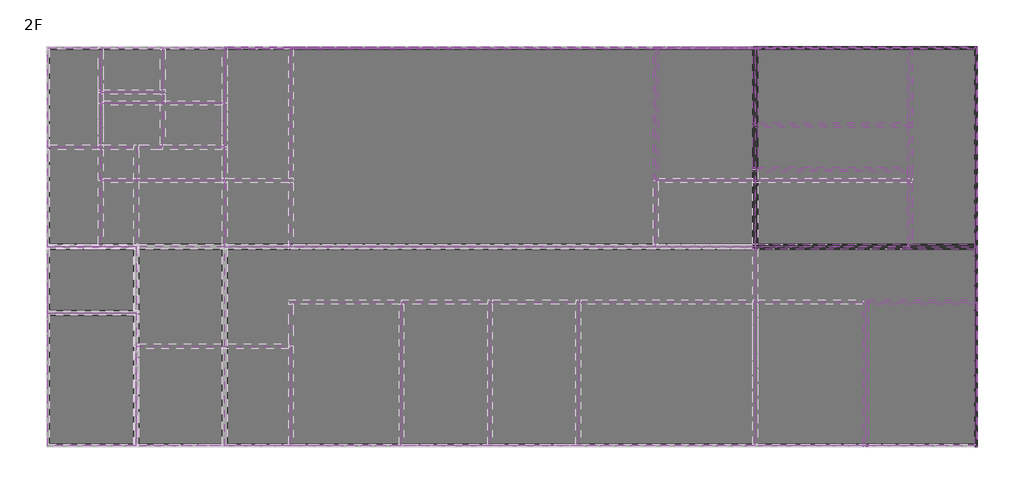
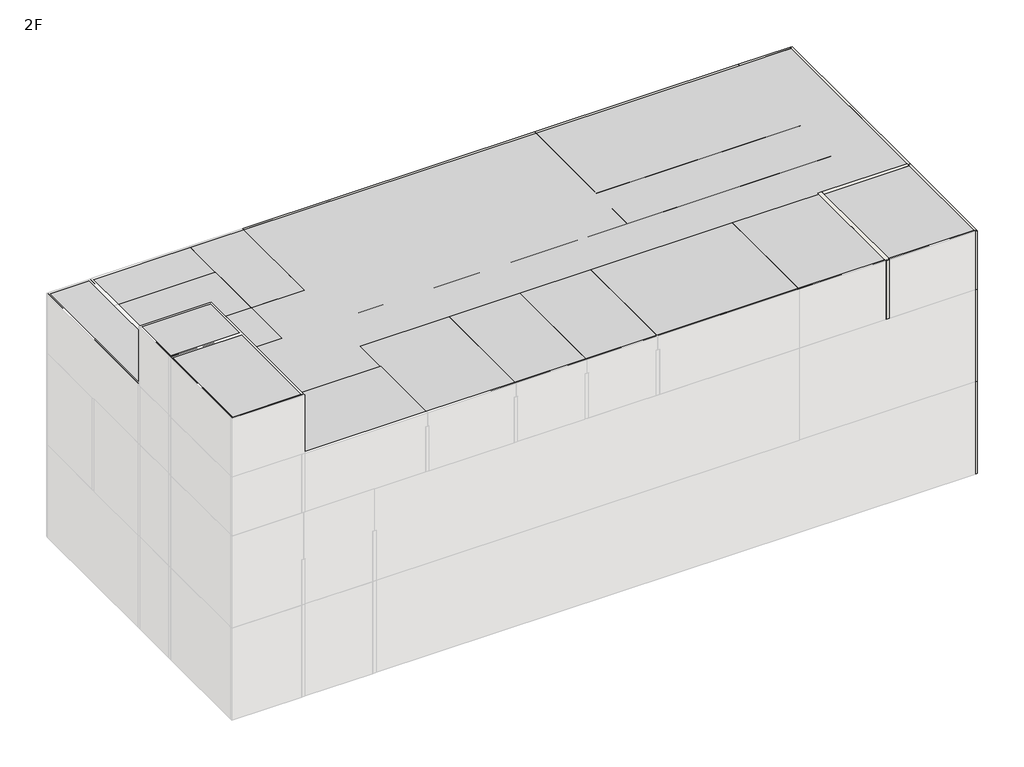
# One storey, part 3 of 3: 39 proxies, 28 walls.
"""IFC4 building model written with IfcOpenShell, lengths in millimetres."""

import ifcopenshell
import ifcopenshell.guid

model = None  # the IFC model being written
_history = None  # IfcOwnerHistory: only IFC2X3 demands one
_inside = {}  # id of a spatial element -> (the spatial element, [elements in it])
_under = {}  # id of a project, library or spatial element -> (it, [spatial elements below it])
_declared = {}  # id of a project -> (the project, [libraries it declares])
_typed = {}  # id of a type object -> (the type object, [elements of that type])
_made_of = {}  # id of a material, layer set ... -> (it, [elements and type objects made of it])


def new_model(schema):
    """Start an empty IFC model of exactly this schema.

    Asked for "IFC4X3", IfcOpenShell would pick the latest addendum, in which some entities
    have other attributes; the version numbers below select the first issue.
    IFC2X3 requires an IfcOwnerHistory on every rooted entity: one is made here for all.
    """
    global model, _history
    if schema == "IFC4X3":
        model = ifcopenshell.file(schema_version=(4, 3, 0, 0))
    else:
        model = ifcopenshell.file(schema=schema)
    _inside.clear()
    _under.clear()
    _declared.clear()
    _typed.clear()
    _made_of.clear()
    _history = None
    if model.schema == "IFC2X3":
        org = make("IfcOrganization", Name="unknown")
        user = make(
            "IfcPersonAndOrganization",
            ThePerson=make("IfcPerson", FamilyName="unknown"),
            TheOrganization=org,
        )
        app = make(
            "IfcApplication",
            ApplicationDeveloper=org,
            Version="unknown",
            ApplicationFullName="unknown",
            ApplicationIdentifier="unknown",
        )
        _history = make(
            "IfcOwnerHistory",
            OwningUser=user,
            OwningApplication=app,
            ChangeAction="ADDED",
            CreationDate=0,
        )
    return model


def make(cls, **values):
    """One entity of the class cls with the attributes given. An attribute that is None is left unset."""
    return model.create_entity(
        cls, **{name: value for name, value in values.items() if value is not None}
    )


def rooted(cls, **values):
    """An entity with a GlobalId (a new one), such as an element, a storey or a relation."""
    return make(cls, GlobalId=ifcopenshell.guid.new(), OwnerHistory=_history, **values)


def si_unit(unit_type, name, prefix=None):
    """IfcSIUnit, for example si_unit("LENGTHUNIT", "METRE", prefix="MILLI")."""
    return make("IfcSIUnit", UnitType=unit_type, Prefix=prefix, Name=name)


def assignment(units):
    """IfcUnitAssignment: the units of a project."""
    return None if units is None else make("IfcUnitAssignment", Units=units)


def point(xyz):
    """IfcCartesianPoint."""
    return None if xyz is None else make("IfcCartesianPoint", Coordinates=xyz)


def direction(xyz):
    """IfcDirection."""
    return None if xyz is None else make("IfcDirection", DirectionRatios=xyz)


def frame(location, z_axis=None, x_axis=None):
    """IfcAxis2Placement3D, a coordinate frame: its origin and axes. An axis left out is left unset."""
    return make(
        "IfcAxis2Placement3D",
        Location=point(location),
        Axis=direction(z_axis),
        RefDirection=direction(x_axis),
    )


def origin():
    """The frame at (0, 0, 0) with its axes left unset."""
    return frame((0.0, 0.0, 0.0))


def origin_with_axes():
    """The frame at (0, 0, 0) with the z axis (0, 0, 1) and the x axis (1, 0, 0) written out."""
    return frame((0.0, 0.0, 0.0), z_axis=(0.0, 0.0, 1.0), x_axis=(1.0, 0.0, 0.0))


def place(relative_to, where):
    """IfcLocalPlacement: puts the frame where relative to a parent placement (None: the world)."""
    return make(
        "IfcLocalPlacement", PlacementRelTo=relative_to, RelativePlacement=where
    )


def context(
    kind, dimensions, precision=None, world=None, true_north=None, identifier=None
):
    """IfcGeometricRepresentationContext, for example the 3D "Model" context."""
    return make(
        "IfcGeometricRepresentationContext",
        ContextIdentifier=identifier,
        ContextType=kind,
        CoordinateSpaceDimension=dimensions,
        Precision=precision,
        WorldCoordinateSystem=world,
        TrueNorth=true_north,
    )


def project(units=None, contexts=None):
    """IfcProject with its units and contexts."""
    return rooted(
        "IfcProject",
        Name="project",
        RepresentationContexts=contexts,
        UnitsInContext=assignment(units),
    )


def spatial(cls, under=None, at=None, **own):
    """A site, building, storey or space (cls), placed at a placement, below another one or the project."""
    s = rooted(cls, ObjectPlacement=at, **own)
    if under is not None:
        _under.setdefault(under.id(), (under, []))[1].append(s)
    return s


def polyline(points):
    """IfcPolyline through the points."""
    return make("IfcPolyline", Points=[point(p) for p in points])


def outline(outer, holes=None, kind="AREA"):
    """IfcArbitraryClosedProfileDef: a profile drawn as a closed curve; with holes, ...WithVoids."""
    if holes is None:
        return make("IfcArbitraryClosedProfileDef", ProfileType=kind, OuterCurve=outer)
    return make(
        "IfcArbitraryProfileDefWithVoids",
        ProfileType=kind,
        OuterCurve=outer,
        InnerCurves=holes,
    )


def extrude(swept, where, along, depth):
    """IfcExtrudedAreaSolid: the profile swept, set in the frame where, extruded along a direction by depth."""
    return make(
        "IfcExtrudedAreaSolid",
        SweptArea=swept,
        Position=where,
        ExtrudedDirection=direction(along),
        Depth=depth,
    )


def faces_of(points, faces, orient=None, outer=None):
    """IfcFace entities. A face is a list of loops; a loop is a list of indices into points, from 0.

    orient and outer hold one flag for each loop. By default every Orientation is true, the
    first loop of a face is its IfcFaceOuterBound and the others are IfcFaceBound.
    """
    made = []
    for i, loops in enumerate(faces):
        bounds = []
        for j, loop in enumerate(loops):
            is_outer = j == 0 if outer is None else outer[i][j]
            bounds.append(
                make(
                    "IfcFaceOuterBound" if is_outer else "IfcFaceBound",
                    Bound=make("IfcPolyLoop", Polygon=[points[k] for k in loop]),
                    Orientation=True if orient is None else orient[i][j],
                )
            )
        made.append(make("IfcFace", Bounds=bounds))
    return made


def faceted_brep(points, faces, orient=None, outer=None, voids=None):
    """IfcFacetedBrep: a solid bounded by flat faces; with voids (closed shells), ...WithVoids."""
    shared = [point(p) for p in points]
    hull = make("IfcClosedShell", CfsFaces=faces_of(shared, faces, orient, outer))
    if voids is None:
        return make("IfcFacetedBrep", Outer=hull)
    return make(
        "IfcFacetedBrepWithVoids",
        Outer=hull,
        Voids=[
            make(cls, CfsFaces=faces_of(shared, fs, o, b)) for cls, fs, o, b in voids
        ],
    )


def shape(context_of_items, identifier, shape_type, items):
    """IfcShapeRepresentation: the items that make up one representation, for example the "Body"."""
    return make(
        "IfcShapeRepresentation",
        ContextOfItems=context_of_items,
        RepresentationIdentifier=identifier,
        RepresentationType=shape_type,
        Items=items,
    )


def source(mapping_origin, context_of_items, identifier, shape_type, items):
    """IfcRepresentationMap: a shape defined once, which mapped items show again and again."""
    return make(
        "IfcRepresentationMap",
        MappingOrigin=mapping_origin,
        MappedRepresentation=shape(context_of_items, identifier, shape_type, items),
    )


def transform(
    local_origin,
    x_axis=None,
    y_axis=None,
    z_axis=None,
    scale=None,
    scale2=None,
    scale3=None,
    uniform=True,
):
    """IfcCartesianTransformationOperator3D, or its non-uniform kind. x_axis, y_axis, z_axis: its Axis1, 2, 3."""
    if uniform:
        return make(
            "IfcCartesianTransformationOperator3D",
            Axis1=direction(x_axis),
            Axis2=direction(y_axis),
            LocalOrigin=point(local_origin),
            Scale=scale,
            Axis3=direction(z_axis),
        )
    return make(
        "IfcCartesianTransformationOperator3DnonUniform",
        Axis1=direction(x_axis),
        Axis2=direction(y_axis),
        LocalOrigin=point(local_origin),
        Scale=scale,
        Axis3=direction(z_axis),
        Scale2=scale2,
        Scale3=scale3,
    )


def mapped(mapping_source, mapping_target):
    """IfcMappedItem: shows the shape of a source again, moved by a transform."""
    return make(
        "IfcMappedItem", MappingSource=mapping_source, MappingTarget=mapping_target
    )


def made_of(thing, what):
    """Note that an element or type object is made of a material, layer set ...; save() writes the relation."""
    if what is not None:
        _made_of.setdefault(what.id(), (what, []))[1].append(thing)
    return thing


def element(
    cls,
    number,
    at=None,
    inside=None,
    cuts=None,
    type_object=None,
    material=None,
    context=None,
    identifier="Body",
    shape_type=None,
    held_by="IfcProductDefinitionShape",
    body=None,
    shapes=None,
    **own,
):
    """One element of the class cls, such as IfcWall. Its Tag is "e" and its number.

    at: its placement. inside: the storey or other place that contains it. cuts: it is an
    opening in that element (IfcRelVoidsElement). A single representation is given by context,
    identifier, shape_type and body (its items); several are given by shapes. held_by: the class
    of the entity that holds the representations. save() writes the other relations.
    """
    e = rooted(cls, Tag="e%d" % number, ObjectPlacement=at, **own)
    if body is not None:
        shapes = [shape(context, identifier, shape_type, body)]
    if shapes is not None:
        e.Representation = make(held_by, Representations=shapes)
    if inside is not None:
        _inside.setdefault(inside.id(), (inside, []))[1].append(e)
    if cuts is not None:
        rooted(
            "IfcRelVoidsElement", RelatingBuildingElement=cuts, RelatedOpeningElement=e
        )
    if type_object is not None:
        _typed.setdefault(type_object.id(), (type_object, []))[1].append(e)
    return made_of(e, material)


def aggregate(whole, parts):
    """IfcRelAggregates: a whole, such as a stair, and the parts it consists of."""
    return rooted("IfcRelAggregates", RelatingObject=whole, RelatedObjects=parts)


def save(model, path):
    """Write the relations noted so far, then the file.

    IfcRelAggregates (storeys below a building ...), IfcRelContainedInSpatialStructure (elements
    in a storey), IfcRelDefinesByType, IfcRelAssociatesMaterial and IfcRelDeclares: one each for
    every whole, place, type object, material and project.
    """
    for whole, parts in _under.values():
        aggregate(whole, parts)
    for where, things in _inside.values():
        rooted(
            "IfcRelContainedInSpatialStructure",
            RelatedElements=things,
            RelatingStructure=where,
        )
    for kind, things in _typed.values():
        rooted("IfcRelDefinesByType", RelatedObjects=things, RelatingType=kind)
    for what, things in _made_of.values():
        rooted("IfcRelAssociatesMaterial", RelatedObjects=things, RelatingMaterial=what)
    for by, libraries in _declared.values():
        rooted("IfcRelDeclares", RelatingContext=by, RelatedDefinitions=libraries)
    model.write(path)


def generic_models_c89eb543(model_context):
    return source(origin(), model_context, "Body", "SweptSolid", [
        extrude(outline(polyline([(2000.0, 3000.0), (2000.0, -3000.0), (-2000.0, -3000.0), (-2000.0, 3000.0), (2000.0, 3000.0)])), origin_with_axes(), (0.0, 0.0, 1.0), 3500.0),
    ])


def generic_models_50f5a469(model_context):
    return source(origin(), model_context, "Body", "SweptSolid", [
        extrude(outline(polyline([(4500.0, 16000.0), (4500.0, -16000.0), (-4500.0, -16000.0), (-4500.0, 16000.0), (4500.0, 16000.0)])), origin_with_axes(), (0.0, 0.0, 1.0), 5500.0),
    ])


def generic_models_8b5775ea(model_context):
    return source(origin(), model_context, "Body", "SweptSolid", [
        extrude(outline(polyline([(4500.0, 17000.0), (4500.0, -17000.0), (-4500.0, -17000.0), (-4500.0, 17000.0), (4500.0, 17000.0)])), origin_with_axes(), (0.0, 0.0, 1.0), 5500.0),
    ])


def generic_models_2d265e4a(model_context):
    return source(origin(), model_context, "Body", "SweptSolid", [
        extrude(outline(polyline([(4500.0, 5000.0), (4500.0, -5000.0), (-4500.0, -5000.0), (-4500.0, 5000.0), (4500.0, 5000.0)])), origin_with_axes(), (0.0, 0.0, 1.0), 5500.0),
    ])


def generic_models_8934d72c(model_context):
    return source(origin(), model_context, "Body", "SweptSolid", [
        extrude(outline(polyline([(2000.0, 4500.0), (2000.0, -4500.0), (-2000.0, -4500.0), (-2000.0, 4500.0), (2000.0, 4500.0)])), origin_with_axes(), (0.0, 0.0, 1.0), 5500.0),
    ])


def generic_models_626d8198(model_context):
    return source(origin(), model_context, "Body", "SweptSolid", [
        extrude(outline(polyline([(2000.0, 1500.0), (2000.0, -1500.0), (-2000.0, -1500.0), (-2000.0, 1500.0), (2000.0, 1500.0)])), origin_with_axes(), (0.0, 0.0, 1.0), 5500.0),
    ])


def generic_models_cc1dae17(model_context):
    return source(origin(), model_context, "Body", "SweptSolid", [
        extrude(outline(polyline([(2000.0, 3000.0), (2000.0, -3000.0), (-2000.0, -3000.0), (-2000.0, 3000.0), (2000.0, 3000.0)])), origin_with_axes(), (0.0, 0.0, 1.0), 5500.0),
    ])


def generic_models_7ea3b148(model_context):
    return source(origin(), model_context, "Body", "SweptSolid", [
        extrude(outline(polyline([(4500.0, 12000.0), (4500.0, -12000.0), (-4500.0, -12000.0), (-4500.0, 12000.0), (4500.0, 12000.0)])), origin_with_axes(), (0.0, 0.0, 1.0), 5500.0),
    ])


def generic_models_85ff21bb(model_context):
    return source(origin(), model_context, "Body", "SweptSolid", [
        extrude(outline(polyline([(3500.0, 1750.0), (3500.0, -1750.0), (-3500.0, -1750.0), (-3500.0, 1750.0), (3500.0, 1750.0)])), origin_with_axes(), (0.0, 0.0, 1.0), 5500.0),
    ])


def generic_models_570012e4(model_context):
    return source(origin(), model_context, "Body", "SweptSolid", [
        extrude(outline(polyline([(1200.0, 2250.0), (1200.0, -2250.0), (-1200.0, -2250.0), (-1200.0, 2250.0), (1200.0, 2250.0)])), origin_with_axes(), (0.0, 0.0, 1.0), 5500.0),
    ])


def generic_models_971c0b89(model_context):
    return source(origin(), model_context, "Body", "SweptSolid", [
        extrude(outline(polyline([(2000.0, 2250.0), (2000.0, -2250.0), (-2000.0, -2250.0), (-2000.0, 2250.0), (2000.0, 2250.0)])), origin_with_axes(), (0.0, 0.0, 1.0), 5500.0),
    ])


def generic_models_ac48a1a3(model_context):
    return source(origin(), model_context, "Body", "SweptSolid", [
        extrude(outline(polyline([(1400.0, 2250.0), (1400.0, -2250.0), (-1400.0, -2250.0), (-1400.0, 2250.0), (1400.0, 2250.0)])), origin_with_axes(), (0.0, 0.0, 1.0), 5500.0),
    ])


def generic_models_ee32b0c6(model_context):
    return source(origin(), model_context, "Body", "SweptSolid", [
        extrude(outline(polyline([(1400.0, 1000.0), (1400.0, -1000.0), (-1400.0, -1000.0), (-1400.0, 1000.0), (1400.0, 1000.0)])), origin_with_axes(), (0.0, 0.0, 1.0), 5500.0),
    ])


def generic_models_0ee3397c(model_context):
    return source(origin(), model_context, "Body", "SweptSolid", [
        extrude(outline(polyline([(1400.0, 1250.0), (1400.0, -1250.0), (-1400.0, -1250.0), (-1400.0, 1250.0), (1400.0, 1250.0)])), origin_with_axes(), (0.0, 0.0, 1.0), 5500.0),
    ])


def generic_models_8c4134a9(model_context):
    return source(origin(), model_context, "Body", "SweptSolid", [
        extrude(outline(polyline([(3250.0, 2000.0), (3250.0, -2000.0), (-3250.0, -2000.0), (-3250.0, 2000.0), (3250.0, 2000.0)])), origin_with_axes(), (0.0, 0.0, 1.0), 3500.0),
    ])


def generic_models_ccc8c8c2(model_context):
    return source(origin(), model_context, "Body", "SweptSolid", [
        extrude(outline(polyline([(3000.0, 5750.0), (3000.0, -5750.0), (-3000.0, -5750.0), (-3000.0, 5750.0), (3000.0, 5750.0)])), origin_with_axes(), (0.0, 0.0, 1.0), 3500.0),
    ])


def generic_models_70f6ae48(model_context):
    return source(origin(), model_context, "Body", "SweptSolid", [
        extrude(outline(polyline([(3250.0, 4000.0), (3250.0, -4000.0), (-3250.0, -4000.0), (-3250.0, 4000.0), (3250.0, 4000.0)])), origin_with_axes(), (0.0, 0.0, 1.0), 3500.0),
    ])


def generic_models_f0561c1d(model_context):
    return source(origin(), model_context, "Body", "SweptSolid", [
        extrude(outline(polyline([(4500.0, 8250.0), (4500.0, -8250.0), (-4500.0, -8250.0), (-4500.0, 8250.0), (4500.0, 8250.0)])), origin_with_axes(), (0.0, 0.0, 1.0), 3500.0),
    ])


def generic_models_249c6621(model_context):
    return source(origin(), model_context, "Body", "SweptSolid", [
        extrude(outline(polyline([(3250.0, 2500.0), (3250.0, -2500.0), (-3250.0, -2500.0), (-3250.0, 2500.0), (3250.0, 2500.0)])), origin_with_axes(), (0.0, 0.0, 1.0), 3500.0),
    ])


def generic_models_f1f4091a(model_context):
    return source(origin(), model_context, "Body", "SweptSolid", [
        extrude(outline(polyline([(1500.0, 5750.0), (1500.0, -5750.0), (-1500.0, -5750.0), (-1500.0, 5750.0), (1500.0, 5750.0)])), origin_with_axes(), (0.0, 0.0, 1.0), 3500.0),
    ])


def generic_models_10b6925f(model_context):
    return source(origin(), model_context, "Body", "SweptSolid", [
        extrude(outline(polyline([(2250.0, 3500.0), (2250.0, -3500.0), (-2250.0, -3500.0), (-2250.0, 3500.0), (2250.0, 3500.0)])), origin_with_axes(), (0.0, 0.0, 1.0), 3500.0),
    ])


def generic_models_b37916ea(model_context):
    return source(origin(), model_context, "Body", "SweptSolid", [
        extrude(outline(polyline([(1750.0, 2800.0), (1750.0, -2800.0), (-1750.0, -2800.0), (-1750.0, 2800.0), (1750.0, 2800.0)])), origin_with_axes(), (0.0, 0.0, 1.0), 3500.0),
    ])


def generic_models_6c75c912(model_context):
    return source(origin(), model_context, "Body", "SweptSolid", [
        extrude(outline(polyline([(1250.0, 2800.0), (1250.0, -2800.0), (-1250.0, -2800.0), (-1250.0, 2800.0), (1250.0, 2800.0)])), origin_with_axes(), (0.0, 0.0, 1.0), 3500.0),
    ])


def generic_models_a5818909(model_context):
    return source(origin(), model_context, "Body", "SweptSolid", [
        extrude(outline(polyline([(3000.0, 1500.0), (3000.0, -1500.0), (-3000.0, -1500.0), (-3000.0, 1500.0), (3000.0, 1500.0)])), origin_with_axes(), (0.0, 0.0, 1.0), 3500.0),
    ])


def generic_models_f42d0df8(model_context):
    return source(origin(), model_context, "Body", "SweptSolid", [
        extrude(outline(polyline([(1500.0, 2800.0), (1500.0, -2800.0), (-1500.0, -2800.0), (-1500.0, 2800.0), (1500.0, 2800.0)])), origin_with_axes(), (0.0, 0.0, 1.0), 3500.0),
    ])


def generic_models_3f6e5246(model_context):
    return source(origin(), model_context, "Body", "SweptSolid", [
        extrude(outline(polyline([(1200.0, 4500.0), (1200.0, -4500.0), (-1200.0, -4500.0), (-1200.0, 4500.0), (1200.0, 4500.0)])), origin_with_axes(), (0.0, 0.0, 1.0), 3500.0),
    ])


def generic_models_4c644d41(model_context):
    return source(origin(), model_context, "Body", "SweptSolid", [
        extrude(outline(polyline([(2000.0, 1500.0), (2000.0, -1500.0), (-2000.0, -1500.0), (-2000.0, 1500.0), (2000.0, 1500.0)])), origin_with_axes(), (0.0, 0.0, 1.0), 3500.0),
    ])


def generic_models_3d03af35(model_context):
    return source(origin(), model_context, "Body", "SweptSolid", [
        extrude(outline(polyline([(21000.0, 9000.0), (21000.0, -9000.0), (-21000.0, -9000.0), (-21000.0, 9000.0), (21000.0, 9000.0)])), origin_with_axes(), (0.0, 0.0, 1.0), 5500.0),
    ])


def generic_models_bb515c93(model_context):
    return source(origin(), model_context, "Body", "SweptSolid", [
        extrude(outline(polyline([(9000.0, 21000.0), (9000.0, -21000.0), (-9000.0, -21000.0), (-9000.0, 21000.0), (9000.0, 21000.0)])), origin_with_axes(), (0.0, 0.0, 1.0), 3500.0),
    ])


model = new_model("IFC4")

# Units and contexts
model_context = context("Model", 3, world=origin())
ifc_project = project(units=[si_unit("LENGTHUNIT", "METRE", prefix="MILLI")], contexts=[model_context])

# Site, building, storey
site = spatial("IfcSite", under=ifc_project)
building = spatial("IfcBuilding", under=site)
storey = spatial("IfcBuildingStorey", under=building, Name="2F", Elevation=3500.0)

# Proxies
placement = place(None, origin())
generic_models_shape = generic_models_c89eb543(model_context)
element("IfcBuildingElementProxy", 1, Name="Space Planning Box_hec : Space Planning Box_hec", ObjectType="Space Planning Box_hec : Space Planning Box_hec", at=placement, inside=storey, context=model_context, shape_type="MappedRepresentation", body=[
    mapped(generic_models_shape, transform((47459.6521483, 166923.8614395, 14500.0), x_axis=(1.0, 0.0, 0.0), y_axis=(0.0, 1.0, 0.0), z_axis=(0.0, 0.0, 1.0))),
])
element("IfcBuildingElementProxy", 2, Name="Space Planning Box_hec : Space Planning Box_hec", ObjectType="Space Planning Box_hec : Space Planning Box_hec", at=placement, inside=storey, context=model_context, shape_type="MappedRepresentation", body=[
    mapped(generic_models_shape, transform((47459.6521483, 166923.8614395, 18000.0), x_axis=(1.0, 0.0, 0.0), y_axis=(0.0, 1.0, 0.0), z_axis=(0.0, 0.0, 1.0))),
])
generic_models_2_shape = generic_models_50f5a469(model_context)
element("IfcBuildingElementProxy", 3, Name="Space Planning Box_hec : Space Planning Box_hec", ObjectType="Space Planning Box_hec : Space Planning Box_hec", at=placement, inside=storey, context=model_context, shape_type="MappedRepresentation", body=[
    mapped(generic_models_2_shape, transform((61459.6521483, 177423.8614395, 3500.0), x_axis=(0.0, 1.0, 0.0), y_axis=(-1.0, 0.0, 0.0), z_axis=(0.0, 0.0, 1.0))),
])
generic_models_3_shape = generic_models_8b5775ea(model_context)
element("IfcBuildingElementProxy", 4, Name="Space Planning Box_hec : Space Planning Box_hec", ObjectType="Space Planning Box_hec : Space Planning Box_hec", at=placement, inside=storey, context=model_context, shape_type="MappedRepresentation", body=[
    mapped(generic_models_3_shape, transform((70459.6521483, 168423.8614395, 3500.0), x_axis=(0.0, 1.0, 0.0), y_axis=(-1.0, 0.0, 0.0), z_axis=(0.0, 0.0, 1.0))),
])
generic_models_4_shape = generic_models_2d265e4a(model_context)
element("IfcBuildingElementProxy", 5, Name="Space Planning Box_hec : Space Planning Box_hec", ObjectType="Space Planning Box_hec : Space Planning Box_hec", at=placement, inside=storey, context=model_context, shape_type="MappedRepresentation", body=[
    mapped(generic_models_4_shape, transform((82459.6521483, 177423.8614395, 3500.0), x_axis=(0.0, 1.0, 0.0), y_axis=(-1.0, 0.0, 0.0), z_axis=(0.0, 0.0, 1.0))),
])
generic_models_5_shape = generic_models_8934d72c(model_context)
element("IfcBuildingElementProxy", 6, Name="Space Planning Box_hec : Space Planning Box_hec", ObjectType="Space Planning Box_hec : Space Planning Box_hec", at=placement, inside=storey, context=model_context, shape_type="MappedRepresentation", body=[
    mapped(generic_models_5_shape, transform((51459.6521483, 168423.8614395, 3500.0), x_axis=(1.0, 0.0, 0.0), y_axis=(0.0, 1.0, 0.0), z_axis=(0.0, 0.0, 1.0))),
])
generic_models_6_shape = generic_models_626d8198(model_context)
element("IfcBuildingElementProxy", 7, Name="Space Planning Box_hec : Space Planning Box_hec", ObjectType="Space Planning Box_hec : Space Planning Box_hec", at=placement, inside=storey, context=model_context, shape_type="MappedRepresentation", body=[
    mapped(generic_models_6_shape, transform((47459.6521483, 171423.8614395, 3500.0), x_axis=(1.0, 0.0, 0.0), y_axis=(0.0, 1.0, 0.0), z_axis=(0.0, 0.0, 1.0))),
])
element("IfcBuildingElementProxy", 8, Name="Space Planning Box_hec : Space Planning Box_hec", ObjectType="Space Planning Box_hec : Space Planning Box_hec", at=placement, inside=storey, context=model_context, shape_type="MappedRepresentation", body=[
    mapped(generic_models_6_shape, transform((47459.6521483, 171423.8614395, 9000.0), x_axis=(1.0, 0.0, 0.0), y_axis=(0.0, 1.0, 0.0), z_axis=(0.0, 0.0, 1.0))),
])
generic_models_7_shape = generic_models_cc1dae17(model_context)
element("IfcBuildingElementProxy", 9, Name="Space Planning Box_hec : Space Planning Box_hec", ObjectType="Space Planning Box_hec : Space Planning Box_hec", at=placement, inside=storey, context=model_context, shape_type="MappedRepresentation", body=[
    mapped(generic_models_7_shape, transform((47459.6521483, 166923.8614395, 3500.0), x_axis=(1.0, 0.0, 0.0), y_axis=(0.0, 1.0, 0.0), z_axis=(0.0, 0.0, 1.0))),
])
element("IfcBuildingElementProxy", 10, Name="Space Planning Box_hec : Space Planning Box_hec", ObjectType="Space Planning Box_hec : Space Planning Box_hec", at=placement, inside=storey, context=model_context, shape_type="MappedRepresentation", body=[
    mapped(generic_models_7_shape, transform((47459.6521483, 166923.8614395, 9000.0), x_axis=(1.0, 0.0, 0.0), y_axis=(0.0, 1.0, 0.0), z_axis=(0.0, 0.0, 1.0))),
])
generic_models_8_shape = generic_models_7ea3b148(model_context)
element("IfcBuildingElementProxy", 11, Name="Space Planning Box_hec : Space Planning Box_hec", ObjectType="Space Planning Box_hec : Space Planning Box_hec", at=placement, inside=storey, context=model_context, shape_type="MappedRepresentation", body=[
    mapped(generic_models_8_shape, transform((65459.6521483, 177423.8614395, 9000.0), x_axis=(0.0, -1.0, 0.0), y_axis=(1.0, 0.0, 0.0), z_axis=(0.0, 0.0, 1.0))),
])
element("IfcBuildingElementProxy", 12, Name="Space Planning Box_hec : Space Planning Box_hec", ObjectType="Space Planning Box_hec : Space Planning Box_hec", at=placement, inside=storey, context=model_context, shape_type="MappedRepresentation", body=[
    mapped(generic_models_8_shape, transform((65459.6521483, 168423.8614395, 9000.0), x_axis=(0.0, -1.0, 0.0), y_axis=(1.0, 0.0, 0.0), z_axis=(0.0, 0.0, 1.0))),
])
generic_models_9_shape = generic_models_85ff21bb(model_context)
element("IfcBuildingElementProxy", 13, Name="Space Planning Box_hec : Space Planning Box_hec", ObjectType="Space Planning Box_hec : Space Planning Box_hec", at=placement, inside=storey, context=model_context, shape_type="MappedRepresentation", body=[
    mapped(generic_models_9_shape, transform((80959.6521483, 180173.8614395, 9000.0), x_axis=(1.0, 0.0, 0.0), y_axis=(0.0, 1.0, 0.0), z_axis=(0.0, 0.0, 1.0))),
])
element("IfcBuildingElementProxy", 14, Name="Space Planning Box_hec : Space Planning Box_hec", ObjectType="Space Planning Box_hec : Space Planning Box_hec", at=placement, inside=storey, context=model_context, shape_type="MappedRepresentation", body=[
    mapped(generic_models_4_shape, transform((82459.6521483, 168423.8614395, 9000.0), x_axis=(0.0, 1.0, 0.0), y_axis=(-1.0, 0.0, 0.0), z_axis=(0.0, 0.0, 1.0))),
])
element("IfcBuildingElementProxy", 15, Name="Space Planning Box_hec : Space Planning Box_hec", ObjectType="Space Planning Box_hec : Space Planning Box_hec", at=placement, inside=storey, context=model_context, shape_type="MappedRepresentation", body=[
    mapped(generic_models_9_shape, transform((80959.6521483, 174673.8614395, 9000.0), x_axis=(1.0, 0.0, 0.0), y_axis=(0.0, 1.0, 0.0), z_axis=(0.0, 0.0, 1.0))),
])
generic_models_10_shape = generic_models_570012e4(model_context)
element("IfcBuildingElementProxy", 16, Name="Space Planning Box_hec : Space Planning Box_hec", ObjectType="Space Planning Box_hec : Space Planning Box_hec", at=placement, inside=storey, context=model_context, shape_type="MappedRepresentation", body=[
    mapped(generic_models_10_shape, transform((46659.6521483, 179673.8614395, 9000.0), x_axis=(1.0, 0.0, 0.0), y_axis=(0.0, 1.0, 0.0), z_axis=(0.0, 0.0, 1.0))),
])
generic_models_11_shape = generic_models_971c0b89(model_context)
element("IfcBuildingElementProxy", 17, Name="Space Planning Box_hec : Space Planning Box_hec", ObjectType="Space Planning Box_hec : Space Planning Box_hec", at=placement, inside=storey, context=model_context, shape_type="MappedRepresentation", body=[
    mapped(generic_models_11_shape, transform((47459.6521483, 175173.8614395, 9000.0), x_axis=(1.0, 0.0, 0.0), y_axis=(0.0, 1.0, 0.0), z_axis=(0.0, 0.0, 1.0))),
])
generic_models_12_shape = generic_models_ac48a1a3(model_context)
element("IfcBuildingElementProxy", 18, Name="Space Planning Box_hec : Space Planning Box_hec", ObjectType="Space Planning Box_hec : Space Planning Box_hec", at=placement, inside=storey, context=model_context, shape_type="MappedRepresentation", body=[
    mapped(generic_models_12_shape, transform((52059.6521483, 179673.8614395, 9000.0), x_axis=(1.0, 0.0, 0.0), y_axis=(0.0, 1.0, 0.0), z_axis=(0.0, 0.0, 1.0))),
])
generic_models_13_shape = generic_models_ee32b0c6(model_context)
element("IfcBuildingElementProxy", 19, Name="Space Planning Box_hec : Space Planning Box_hec", ObjectType="Space Planning Box_hec : Space Planning Box_hec", at=placement, inside=storey, context=model_context, shape_type="MappedRepresentation", body=[
    mapped(generic_models_13_shape, transform((49259.6521483, 180923.8614395, 9000.0), x_axis=(1.0, 0.0, 0.0), y_axis=(0.0, 1.0, 0.0), z_axis=(0.0, 0.0, 1.0))),
])
generic_models_14_shape = generic_models_0ee3397c(model_context)
element("IfcBuildingElementProxy", 20, Name="Space Planning Box_hec : Space Planning Box_hec", ObjectType="Space Planning Box_hec : Space Planning Box_hec", at=placement, inside=storey, context=model_context, shape_type="MappedRepresentation", body=[
    mapped(generic_models_14_shape, transform((49259.6521483, 178673.8614395, 9000.0), x_axis=(1.0, 0.0, 0.0), y_axis=(0.0, 1.0, 0.0), z_axis=(0.0, 0.0, 1.0))),
])
generic_models_15_shape = generic_models_8c4134a9(model_context)
element("IfcBuildingElementProxy", 21, Name="Space Planning Box_hec : Space Planning Box_hec", ObjectType="Space Planning Box_hec : Space Planning Box_hec", at=placement, inside=storey, context=model_context, shape_type="MappedRepresentation", body=[
    mapped(generic_models_15_shape, transform((63459.6521483, 167173.8614395, 14500.0), x_axis=(0.0, 1.0, 0.0), y_axis=(-1.0, 0.0, 0.0), z_axis=(0.0, 0.0, 1.0))),
])
element("IfcBuildingElementProxy", 22, Name="Space Planning Box_hec : Space Planning Box_hec", ObjectType="Space Planning Box_hec : Space Planning Box_hec", at=placement, inside=storey, context=model_context, shape_type="MappedRepresentation", body=[
    mapped(generic_models_15_shape, transform((67459.6521483, 167173.8614395, 14500.0), x_axis=(0.0, 1.0, 0.0), y_axis=(-1.0, 0.0, 0.0), z_axis=(0.0, 0.0, 1.0))),
])
generic_models_16_shape = generic_models_ccc8c8c2(model_context)
element("IfcBuildingElementProxy", 23, Name="Space Planning Box_hec : Space Planning Box_hec", ObjectType="Space Planning Box_hec : Space Planning Box_hec", at=placement, inside=storey, context=model_context, shape_type="MappedRepresentation", body=[
    mapped(generic_models_16_shape, transform((78709.6521483, 178923.8614395, 14500.0), x_axis=(0.0, -1.0, 0.0), y_axis=(1.0, 0.0, 0.0), z_axis=(0.0, 0.0, 1.0))),
])
generic_models_17_shape = generic_models_70f6ae48(model_context)
element("IfcBuildingElementProxy", 24, Name="Space Planning Box_hec : Space Planning Box_hec", ObjectType="Space Planning Box_hec : Space Planning Box_hec", at=placement, inside=storey, context=model_context, shape_type="MappedRepresentation", body=[
    mapped(generic_models_17_shape, transform((73459.6521483, 167173.8614395, 14500.0), x_axis=(0.0, -1.0, 0.0), y_axis=(1.0, 0.0, 0.0), z_axis=(0.0, 0.0, 1.0))),
])
generic_models_18_shape = generic_models_f0561c1d(model_context)
element("IfcBuildingElementProxy", 25, Name="Space Planning Box_hec : Space Planning Box_hec", ObjectType="Space Planning Box_hec : Space Planning Box_hec", at=placement, inside=storey, context=model_context, shape_type="MappedRepresentation", body=[
    mapped(generic_models_18_shape, transform((64709.6521483, 177423.8614395, 14500.0), x_axis=(0.0, -1.0, 0.0), y_axis=(1.0, 0.0, 0.0), z_axis=(0.0, 0.0, 1.0))),
])
generic_models_19_shape = generic_models_249c6621(model_context)
element("IfcBuildingElementProxy", 26, Name="Space Planning Box_hec : Space Planning Box_hec", ObjectType="Space Planning Box_hec : Space Planning Box_hec", at=placement, inside=storey, context=model_context, shape_type="MappedRepresentation", body=[
    mapped(generic_models_19_shape, transform((79959.6521483, 167173.8614395, 14500.0), x_axis=(0.0, -1.0, 0.0), y_axis=(1.0, 0.0, 0.0), z_axis=(0.0, 0.0, 1.0))),
])
element("IfcBuildingElementProxy", 27, Name="Space Planning Box_hec : Space Planning Box_hec", ObjectType="Space Planning Box_hec : Space Planning Box_hec", at=placement, inside=storey, context=model_context, shape_type="MappedRepresentation", body=[
    mapped(generic_models_19_shape, transform((58959.6521483, 167173.8614395, 14500.0), x_axis=(0.0, 1.0, 0.0), y_axis=(-1.0, 0.0, 0.0), z_axis=(0.0, 0.0, 1.0))),
])
element("IfcBuildingElementProxy", 28, Name="Space Planning Box_hec : Space Planning Box_hec", ObjectType="Space Planning Box_hec : Space Planning Box_hec", at=placement, inside=storey, context=model_context, shape_type="MappedRepresentation", body=[
    mapped(generic_models_19_shape, transform((84959.6521483, 167173.8614395, 14500.0), x_axis=(0.0, 1.0, 0.0), y_axis=(-1.0, 0.0, 0.0), z_axis=(0.0, 0.0, 1.0))),
])
generic_models_20_shape = generic_models_f1f4091a(model_context)
element("IfcBuildingElementProxy", 29, Name="Space Planning Box_hec : Space Planning Box_hec", ObjectType="Space Planning Box_hec : Space Planning Box_hec", at=placement, inside=storey, context=model_context, shape_type="MappedRepresentation", body=[
    mapped(generic_models_20_shape, transform((78709.6521483, 174423.8614395, 14500.0), x_axis=(0.0, 1.0, 0.0), y_axis=(-1.0, 0.0, 0.0), z_axis=(0.0, 0.0, 1.0))),
])
generic_models_21_shape = generic_models_10b6925f(model_context)
element("IfcBuildingElementProxy", 30, Name="Space Planning Box_hec : Space Planning Box_hec", ObjectType="Space Planning Box_hec : Space Planning Box_hec", at=placement, inside=storey, context=model_context, shape_type="MappedRepresentation", body=[
    mapped(generic_models_21_shape, transform((52959.6521483, 166173.8614395, 14500.0), x_axis=(0.0, -1.0, 0.0), y_axis=(1.0, 0.0, 0.0), z_axis=(0.0, 0.0, 1.0))),
])
generic_models_22_shape = generic_models_b37916ea(model_context)
element("IfcBuildingElementProxy", 31, Name="Space Planning Box_hec : Space Planning Box_hec", ObjectType="Space Planning Box_hec : Space Planning Box_hec", at=placement, inside=storey, context=model_context, shape_type="MappedRepresentation", body=[
    mapped(generic_models_22_shape, transform((50659.6521483, 177673.8614395, 14500.0), x_axis=(0.0, -1.0, 0.0), y_axis=(1.0, 0.0, 0.0), z_axis=(0.0, 0.0, 1.0))),
])
generic_models_23_shape = generic_models_6c75c912(model_context)
element("IfcBuildingElementProxy", 32, Name="Space Planning Box_hec : Space Planning Box_hec", ObjectType="Space Planning Box_hec : Space Planning Box_hec", at=placement, inside=storey, context=model_context, shape_type="MappedRepresentation", body=[
    mapped(generic_models_23_shape, transform((50659.6521483, 180673.8614395, 14500.0), x_axis=(0.0, -1.0, 0.0), y_axis=(1.0, 0.0, 0.0), z_axis=(0.0, 0.0, 1.0))),
])
generic_models_24_shape = generic_models_a5818909(model_context)
element("IfcBuildingElementProxy", 33, Name="Space Planning Box_hec : Space Planning Box_hec", ObjectType="Space Planning Box_hec : Space Planning Box_hec", at=placement, inside=storey, context=model_context, shape_type="MappedRepresentation", body=[
    mapped(generic_models_24_shape, transform((54959.6521483, 178923.8614395, 14500.0), x_axis=(0.0, -1.0, 0.0), y_axis=(1.0, 0.0, 0.0), z_axis=(0.0, 0.0, 1.0))),
])
generic_models_25_shape = generic_models_f42d0df8(model_context)
element("IfcBuildingElementProxy", 34, Name="Space Planning Box_hec : Space Planning Box_hec", ObjectType="Space Planning Box_hec : Space Planning Box_hec", at=placement, inside=storey, context=model_context, shape_type="MappedRepresentation", body=[
    mapped(generic_models_25_shape, transform((50659.6521483, 174423.8614395, 14500.0), x_axis=(0.0, -1.0, 0.0), y_axis=(1.0, 0.0, 0.0), z_axis=(0.0, 0.0, 1.0))),
])
generic_models_26_shape = generic_models_3f6e5246(model_context)
element("IfcBuildingElementProxy", 35, Name="Space Planning Box_hec : Space Planning Box_hec", ObjectType="Space Planning Box_hec : Space Planning Box_hec", at=placement, inside=storey, context=model_context, shape_type="MappedRepresentation", body=[
    mapped(generic_models_26_shape, transform((46659.6521483, 177423.8614395, 14500.0), x_axis=(1.0, 0.0, 0.0), y_axis=(0.0, 1.0, 0.0), z_axis=(0.0, 0.0, 1.0))),
])
generic_models_27_shape = generic_models_4c644d41(model_context)
element("IfcBuildingElementProxy", 36, Name="Space Planning Box_hec : Space Planning Box_hec", ObjectType="Space Planning Box_hec : Space Planning Box_hec", at=placement, inside=storey, context=model_context, shape_type="MappedRepresentation", body=[
    mapped(generic_models_27_shape, transform((47459.6521483, 171423.8614395, 14500.0), x_axis=(1.0, 0.0, 0.0), y_axis=(0.0, 1.0, 0.0), z_axis=(0.0, 0.0, 1.0))),
])
element("IfcBuildingElementProxy", 37, Name="Space Planning Box_hec : Space Planning Box_hec", ObjectType="Space Planning Box_hec : Space Planning Box_hec", at=placement, inside=storey, context=model_context, shape_type="MappedRepresentation", body=[
    mapped(generic_models_27_shape, transform((47459.6521483, 171423.8614395, 18000.0), x_axis=(1.0, 0.0, 0.0), y_axis=(0.0, 1.0, 0.0), z_axis=(0.0, 0.0, 1.0))),
])
generic_models_28_shape = generic_models_3d03af35(model_context)
element("IfcBuildingElementProxy", 38, Name="Space Planning Box_hec : Space Planning Box_hec", ObjectType="Space Planning Box_hec : Space Planning Box_hec", at=placement, inside=storey, context=model_context, shape_type="MappedRepresentation", body=[
    mapped(generic_models_28_shape, transform((66459.6521483, 172923.8614395, 9000.0), x_axis=(1.0, 0.0, 0.0), y_axis=(0.0, 1.0, 0.0), z_axis=(0.0, 0.0, 1.0))),
])
generic_models_29_shape = generic_models_bb515c93(model_context)
element("IfcBuildingElementProxy", 39, Name="Space Planning Box_hec : Space Planning Box_hec", ObjectType="Space Planning Box_hec : Space Planning Box_hec", at=placement, inside=storey, context=model_context, shape_type="MappedRepresentation", body=[
    mapped(generic_models_29_shape, transform((66459.6521483, 172923.8614395, 14500.0), x_axis=(0.0, -1.0, 0.0), y_axis=(1.0, 0.0, 0.0), z_axis=(0.0, 0.0, 1.0))),
])

# Walls
element("IfcWall", 40, ObjectType="WA211_Exterior-Cement Brick-90mm", at=placement, inside=storey, context=model_context, shape_type="Brep", body=[
    faceted_brep([(87402.6521483, 172923.8614395, 3500.0), (87402.6521483, 172816.8614395, 3500.0), (87402.6521483, 163980.8614395, 3500.0), (87402.6521483, 163866.8614395, 3500.0), (87402.6521483, 163866.8614395, 9000.0), (87402.6521483, 163980.8614395, 9000.0), (87402.6521483, 172816.8614395, 9000.0), (87402.6521483, 172923.8614395, 9000.0), (87516.6521483, 172923.8614395, 3500.0), (87516.6521483, 172923.8614395, 9000.0), (87516.6521483, 163866.8614395, 9000.0), (87516.6521483, 163866.8614395, 3500.0)], [[[0, 1, 2, 3, 4, 5, 6, 7]], [[8, 9, 10, 11]], [[3, 2, 1, 0, 8, 11]], [[7, 6, 5, 4, 10, 9]], [[0, 7, 9, 8]], [[4, 3, 11, 10]]]),
])
element("IfcWall", 41, ObjectType="WA211_Exterior-Cement Brick-90mm", at=placement, inside=storey, context=model_context, shape_type="Brep", body=[
    faceted_brep([(87402.6521483, 181980.8614395, 3500.0), (87402.6521483, 181866.8614395, 3500.0), (87402.6521483, 173030.8614395, 3500.0), (87402.6521483, 172923.8614395, 3500.0), (87402.6521483, 172923.8614395, 9000.0), (87402.6521483, 173030.8614395, 9000.0), (87402.6521483, 181866.8614395, 9000.0), (87402.6521483, 181980.8614395, 9000.0), (87516.6521483, 181980.8614395, 3500.0), (87516.6521483, 181980.8614395, 9000.0), (87516.6521483, 172923.8614395, 9000.0), (87516.6521483, 172923.8614395, 3500.0)], [[[0, 1, 2, 3, 4, 5, 6, 7]], [[8, 9, 10, 11]], [[3, 2, 1, 0, 8, 11]], [[4, 3, 11, 10]], [[7, 6, 5, 4, 10, 9]], [[0, 7, 9, 8]]]),
])
element("IfcWall", 42, ObjectType="WA211_Exterior-Cement Brick-90mm", at=placement, inside=storey, context=model_context, shape_type="SweptSolid", body=[
    extrude(outline(polyline([(87402.6521483, 181866.8614395), (77566.6521483, 181866.8614395), (77566.6521483, 181980.8614395), (87402.6521483, 181980.8614395), (87402.6521483, 181866.8614395)])), frame((0.0, 0.0, 3500.0), z_axis=(0.0, 0.0, 1.0), x_axis=(1.0, 0.0, 0.0)), (0.0, 0.0, 1.0), 5500.0),
])
element("IfcWall", 43, ObjectType="WA211_Exterior-Cement Brick-90mm", at=placement, inside=storey, context=model_context, shape_type="SweptSolid", body=[
    extrude(outline(polyline([(9000.0, 53566.6521483), (9000.0, 77352.6521483), (12400.0, 77352.6521483), (12400.0, 77459.6521483), (14500.0, 77459.6521483), (14500.0, 53459.6521483), (12400.0, 53459.6521483), (12400.0, 53566.6521483), (9000.0, 53566.6521483)])), frame((0.0, 181866.8614395, 0.0), z_axis=(0.0, 1.0, 0.0), x_axis=(0.0, 0.0, 1.0)), (0.0, 0.0, 1.0), 114.0),
])
element("IfcWall", 44, ObjectType="WA211_Exterior-Cement Brick-90mm", at=placement, inside=storey, context=model_context, shape_type="SweptSolid", body=[
    extrude(outline(polyline([(9000.0, 77566.6521483), (9000.0, 84352.6521483), (11700.0, 84352.6521483), (11700.0, 84459.6521483), (14500.0, 84459.6521483), (14500.0, 77459.6521483), (12400.0, 77459.6521483), (12400.0, 77566.6521483), (9000.0, 77566.6521483)])), frame((0.0, 181866.8614395, 0.0), z_axis=(0.0, 1.0, 0.0), x_axis=(0.0, 0.0, 1.0)), (0.0, 0.0, 1.0), 114.0),
])
element("IfcWall", 45, ObjectType="WA211_Exterior-Cement Brick-90mm", at=placement, inside=storey, context=model_context, shape_type="Brep", body=[
    faceted_brep([(87402.6521483, 172923.8614395, 9000.0), (87402.6521483, 172816.8614395, 9000.0), (87402.6521483, 163980.8614395, 9000.0), (87402.6521483, 163866.8614395, 9000.0), (87402.6521483, 163866.8614395, 14500.0), (87402.6521483, 163980.8614395, 14500.0), (87402.6521483, 172816.8614395, 14500.0), (87402.6521483, 172923.8614395, 14500.0), (87516.6521483, 172923.8614395, 9000.0), (87516.6521483, 172923.8614395, 14500.0), (87516.6521483, 163866.8614395, 14500.0), (87516.6521483, 163866.8614395, 9000.0)], [[[0, 1, 2, 3, 4, 5, 6, 7]], [[8, 9, 10, 11]], [[3, 2, 1, 0, 8, 11]], [[7, 6, 5, 4, 10, 9]], [[0, 7, 9, 8]], [[4, 3, 11, 10]]]),
])
element("IfcWall", 46, ObjectType="WA211_Exterior-Cement Brick-90mm", at=placement, inside=storey, context=model_context, shape_type="Brep", body=[
    faceted_brep([(87402.6521483, 181980.8614395, 9000.0), (87402.6521483, 181866.8614395, 9000.0), (87402.6521483, 173030.8614395, 9000.0), (87402.6521483, 172923.8614395, 9000.0), (87402.6521483, 172923.8614395, 14500.0), (87402.6521483, 173030.8614395, 14500.0), (87402.6521483, 181866.8614395, 14500.0), (87402.6521483, 181980.8614395, 14500.0), (87516.6521483, 181980.8614395, 9000.0), (87516.6521483, 181980.8614395, 14500.0), (87516.6521483, 172923.8614395, 14500.0), (87516.6521483, 172923.8614395, 9000.0)], [[[0, 1, 2, 3, 4, 5, 6, 7]], [[8, 9, 10, 11]], [[3, 2, 1, 0, 8, 11]], [[4, 3, 11, 10]], [[7, 6, 5, 4, 10, 9]], [[0, 7, 9, 8]]]),
])
element("IfcWall", 47, ObjectType="WA211_Exterior-Cement Brick-90mm", at=placement, inside=storey, context=model_context, shape_type="SweptSolid", body=[
    extrude(outline(polyline([(9000.0, 84566.6521483), (9000.0, 87402.6521483), (14500.0, 87402.6521483), (14500.0, 84459.6521483), (11700.0, 84459.6521483), (11700.0, 84566.6521483), (9000.0, 84566.6521483)])), frame((0.0, 181866.8614395, 0.0), z_axis=(0.0, 1.0, 0.0), x_axis=(0.0, 0.0, 1.0)), (0.0, 0.0, 1.0), 114.0),
])
element("IfcWall", 48, ObjectType="WA211_Exterior-Cement Brick-90mm", at=placement, inside=storey, context=model_context, shape_type="SweptSolid", body=[
    extrude(outline(polyline([(14500.0, 73066.6521483), (14500.0, 84352.6521483), (17200.0, 84352.6521483), (17200.0, 84459.6521483), (18000.0, 84459.6521483), (18000.0, 72959.6521483), (17200.0, 72959.6521483), (17200.0, 73066.6521483), (14500.0, 73066.6521483)])), frame((0.0, 181866.8614395, 0.0), z_axis=(0.0, 1.0, 0.0), x_axis=(0.0, 0.0, 1.0)), (0.0, 0.0, 1.0), 114.0),
])
element("IfcWall", 49, ObjectType="WA211_Exterior-Cement Brick-90mm", at=placement, inside=storey, context=model_context, shape_type="SweptSolid", body=[
    extrude(outline(polyline([(14500.0, 56566.6521483), (14500.0, 72852.6521483), (17200.0, 72852.6521483), (17200.0, 72959.6521483), (18000.0, 72959.6521483), (18000.0, 56459.6521483), (17200.0, 56459.6521483), (17200.0, 56566.6521483), (14500.0, 56566.6521483)])), frame((0.0, 181866.8614395, 0.0), z_axis=(0.0, 1.0, 0.0), x_axis=(0.0, 0.0, 1.0)), (0.0, 0.0, 1.0), 114.0),
])
element("IfcWall", 50, ObjectType="WA211_Exterior-Cement Brick-90mm", at=placement, inside=storey, context=model_context, shape_type="Brep", body=[
    faceted_brep([(87402.6521483, 170423.8614395, 14500.0), (87402.6521483, 170316.8614395, 14500.0), (87402.6521483, 163980.8614395, 14500.0), (87402.6521483, 163866.8614395, 14500.0), (87402.6521483, 163866.8614395, 18000.0), (87402.6521483, 163980.8614395, 18000.0), (87402.6521483, 170316.8614395, 18000.0), (87402.6521483, 170423.8614395, 18000.0), (87516.6521483, 170423.8614395, 14500.0), (87516.6521483, 170423.8614395, 18000.0), (87516.6521483, 163866.8614395, 18000.0), (87516.6521483, 163866.8614395, 14500.0)], [[[0, 1, 2, 3, 4, 5, 6, 7]], [[8, 9, 10, 11]], [[3, 2, 1, 0, 8, 11]], [[7, 6, 5, 4, 10, 9]], [[0, 7, 9, 8]], [[4, 3, 11, 10]]]),
])
element("IfcWall", 51, ObjectType="WA211_Exterior-Cement Brick-90mm", at=placement, inside=storey, context=model_context, shape_type="Brep", body=[
    faceted_brep([(87402.6521483, 181980.8614395, 14500.0), (87402.6521483, 181866.8614395, 14500.0), (87402.6521483, 170530.8614395, 14500.0), (87402.6521483, 170423.8614395, 14500.0), (87402.6521483, 170423.8614395, 18000.0), (87402.6521483, 170530.8614395, 18000.0), (87402.6521483, 181866.8614395, 18000.0), (87402.6521483, 181980.8614395, 18000.0), (87516.6521483, 181980.8614395, 14500.0), (87516.6521483, 181980.8614395, 18000.0), (87516.6521483, 170423.8614395, 18000.0), (87516.6521483, 170423.8614395, 14500.0)], [[[0, 1, 2, 3, 4, 5, 6, 7]], [[8, 9, 10, 11]], [[3, 2, 1, 0, 8, 11]], [[4, 3, 11, 10]], [[7, 6, 5, 4, 10, 9]], [[0, 7, 9, 8]]]),
])
element("IfcWall", 52, ObjectType="WA211_Exterior-Cement Brick-90mm", at=placement, inside=storey, context=model_context, shape_type="SweptSolid", body=[
    extrude(outline(polyline([(14500.0, 84566.6521483), (14500.0, 87402.6521483), (18000.0, 87402.6521483), (18000.0, 84459.6521483), (17200.0, 84459.6521483), (17200.0, 84566.6521483), (14500.0, 84566.6521483)])), frame((0.0, 181866.8614395, 0.0), z_axis=(0.0, 1.0, 0.0), x_axis=(0.0, 0.0, 1.0)), (0.0, 0.0, 1.0), 114.0),
])
element("IfcWall", 53, ObjectType="WA221_Interior-Cement Block-190mm", at=placement, inside=storey, context=model_context, shape_type="Brep", body=[
    faceted_brep([(77566.6521483, 172816.8614395, 3500.0), (77566.6521483, 173030.8614395, 3500.0), (77566.6521483, 181866.8614395, 3500.0), (77566.6521483, 181980.8614395, 3500.0), (77566.6521483, 181980.8614395, 9000.0), (77566.6521483, 181866.8614395, 9000.0), (77566.6521483, 173030.8614395, 9000.0), (77566.6521483, 172816.8614395, 9000.0), (77352.6521483, 172816.8614395, 3500.0), (77352.6521483, 172816.8614395, 9000.0), (77352.6521483, 173030.8614395, 9000.0), (77352.6521483, 181866.8614395, 9000.0), (77352.6521483, 181980.8614395, 9000.0), (77352.6521483, 181980.8614395, 3500.0), (77352.6521483, 181866.8614395, 3500.0), (77352.6521483, 173030.8614395, 3500.0)], [[[0, 1, 2, 3, 4, 5, 6, 7]], [[8, 9, 10, 11, 12, 13, 14, 15]], [[3, 2, 1, 0, 8, 15, 14, 13]], [[7, 6, 5, 4, 12, 11, 10, 9]], [[0, 7, 9, 8]], [[4, 3, 13, 12]]]),
])
element("IfcWall", 54, ObjectType="WA221_Interior-Cement Block-190mm", at=placement, inside=storey, context=model_context, shape_type="Brep", body=[
    faceted_brep([(77566.6521483, 172816.8614395, 3500.0), (87402.6521483, 172816.8614395, 3500.0), (87402.6521483, 172816.8614395, 9000.0), (77566.6521483, 172816.8614395, 9000.0), (77566.6521483, 173030.8614395, 3500.0), (77566.6521483, 173030.8614395, 9000.0), (87402.6521483, 173030.8614395, 9000.0), (87402.6521483, 173030.8614395, 3500.0), (87402.6521483, 172923.8614395, 3500.0), (87402.6521483, 172923.8614395, 9000.0)], [[[0, 1, 2, 3]], [[4, 5, 6, 7]], [[1, 0, 4, 7, 8]], [[3, 2, 9, 6, 5]], [[0, 3, 5, 4]], [[2, 1, 8, 7, 6, 9]]]),
])
element("IfcWall", 55, ObjectType="WA221_Interior-Cement Block-190mm", at=placement, inside=storey, context=model_context, shape_type="Brep", body=[
    faceted_brep([(77352.6521483, 181980.8614395, 9000.0), (77352.6521483, 181866.8614395, 9000.0), (77352.6521483, 178530.8614395, 9000.0), (77352.6521483, 178530.8614395, 11700.0), (77352.6521483, 178423.8614395, 11700.0), (77352.6521483, 178423.8614395, 12400.0), (77352.6521483, 181866.8614395, 12400.0), (77352.6521483, 181980.8614395, 12400.0), (77566.6521483, 181980.8614395, 9000.0), (77566.6521483, 181980.8614395, 12400.0), (77566.6521483, 181866.8614395, 12400.0), (77566.6521483, 178423.8614395, 12400.0), (77566.6521483, 178423.8614395, 11700.0), (77566.6521483, 178530.8614395, 11700.0), (77566.6521483, 178530.8614395, 9000.0), (77566.6521483, 181866.8614395, 9000.0), (77459.6521483, 181980.8614395, 12400.0)], [[[0, 1, 2, 3, 4, 5, 6, 7]], [[8, 9, 10, 11, 12, 13, 14, 15]], [[2, 1, 0, 8, 15, 14]], [[7, 6, 5, 11, 10, 9, 16]], [[0, 7, 16, 9, 8]], [[5, 4, 12, 11]], [[12, 4, 3, 13]], [[3, 2, 14, 13]]]),
])
element("IfcWall", 56, ObjectType="WA221_Interior-Cement Block-190mm", at=placement, inside=storey, context=model_context, shape_type="SweptSolid", body=[
    extrude(outline(polyline([(178316.8614395, 9000.0), (176530.8614395, 9000.0), (176530.8614395, 11700.0), (176423.8614395, 11700.0), (176423.8614395, 12400.0), (178423.8614395, 12400.0), (178423.8614395, 11700.0), (178316.8614395, 11700.0), (178316.8614395, 9000.0)])), frame((77352.6521483, 0.0, 0.0), z_axis=(1.0, 0.0, 0.0), x_axis=(0.0, 1.0, 0.0)), (0.0, 0.0, 1.0), 214.0),
])
element("IfcWall", 57, ObjectType="WA221_Interior-Cement Block-190mm", at=placement, inside=storey, context=model_context, shape_type="Brep", body=[
    faceted_brep([(84566.6521483, 178530.8614395, 9000.0), (84352.6521483, 178530.8614395, 9000.0), (77566.6521483, 178530.8614395, 9000.0), (77352.6521483, 178530.8614395, 9000.0), (77352.6521483, 178530.8614395, 11700.0), (77566.6521483, 178530.8614395, 11700.0), (84352.6521483, 178530.8614395, 11700.0), (84566.6521483, 178530.8614395, 11700.0), (84566.6521483, 178316.8614395, 9000.0), (84566.6521483, 178316.8614395, 11700.0), (77566.6521483, 178316.8614395, 11700.0), (77352.6521483, 178316.8614395, 11700.0), (77352.6521483, 178316.8614395, 9000.0), (77566.6521483, 178316.8614395, 9000.0), (77352.6521483, 178423.8614395, 11700.0)], [[[0, 1, 2, 3, 4, 5, 6, 7]], [[8, 9, 10, 11, 12, 13]], [[3, 2, 1, 0, 8, 13, 12]], [[7, 6, 5, 4, 14, 11, 10, 9]], [[4, 3, 12, 11, 14]], [[0, 7, 9, 8]]]),
])
element("IfcWall", 58, ObjectType="WA221_Interior-Cement Block-190mm", at=placement, inside=storey, context=model_context, shape_type="Brep", body=[
    faceted_brep([(84352.6521483, 181980.8614395, 9000.0), (84352.6521483, 181866.8614395, 9000.0), (84352.6521483, 178530.8614395, 9000.0), (84352.6521483, 178530.8614395, 11700.0), (84352.6521483, 181866.8614395, 11700.0), (84352.6521483, 181980.8614395, 11700.0), (84566.6521483, 181980.8614395, 9000.0), (84566.6521483, 181980.8614395, 11700.0), (84566.6521483, 181866.8614395, 11700.0), (84566.6521483, 178530.8614395, 11700.0), (84566.6521483, 178530.8614395, 9000.0), (84566.6521483, 181866.8614395, 9000.0), (84459.6521483, 181980.8614395, 11700.0)], [[[0, 1, 2, 3, 4, 5]], [[6, 7, 8, 9, 10, 11]], [[2, 1, 0, 6, 11, 10]], [[5, 4, 3, 9, 8, 7, 12]], [[0, 5, 12, 7, 6]], [[3, 2, 10, 9]]]),
])
element("IfcWall", 59, ObjectType="WA221_Interior-Cement Block-190mm", at=placement, inside=storey, context=model_context, shape_type="Brep", body=[
    faceted_brep([(77459.6521483, 172816.8614395, 9000.0), (77566.6521483, 172816.8614395, 9000.0), (84459.6521483, 172816.8614395, 9000.0), (84459.6521483, 172816.8614395, 14500.0), (77566.6521483, 172816.8614395, 14500.0), (77352.6521483, 172816.8614395, 14500.0), (77352.6521483, 172816.8614395, 12400.0), (77459.6521483, 172816.8614395, 12400.0), (77459.6521483, 173030.8614395, 9000.0), (77459.6521483, 173030.8614395, 12400.0), (77352.6521483, 173030.8614395, 12400.0), (77352.6521483, 173030.8614395, 14500.0), (84459.6521483, 173030.8614395, 14500.0), (84459.6521483, 173030.8614395, 9000.0), (84352.6521483, 173030.8614395, 9000.0), (77566.6521483, 173030.8614395, 9000.0)], [[[0, 1, 2, 3, 4, 5, 6, 7]], [[8, 9, 10, 11, 12, 13, 14, 15]], [[2, 1, 0, 8, 15, 14, 13]], [[5, 4, 3, 12, 11]], [[0, 7, 9, 8]], [[6, 10, 9, 7]], [[6, 5, 11, 10]], [[2, 13, 12, 3]]]),
])
element("IfcWall", 60, ObjectType="WA221_Interior-Cement Block-190mm", at=placement, inside=storey, context=model_context, shape_type="Brep", body=[
    faceted_brep([(84459.6521483, 172816.8614395, 14500.0), (84459.6521483, 172816.8614395, 9000.0), (87402.6521483, 172816.8614395, 9000.0), (87402.6521483, 172816.8614395, 14500.0), (84459.6521483, 173030.8614395, 9000.0), (84459.6521483, 173030.8614395, 14500.0), (87402.6521483, 173030.8614395, 14500.0), (87402.6521483, 173030.8614395, 9000.0), (84566.6521483, 173030.8614395, 9000.0), (87402.6521483, 172923.8614395, 9000.0), (87402.6521483, 172923.8614395, 14500.0)], [[[0, 1, 2, 3]], [[4, 5, 6, 7, 8]], [[2, 1, 4, 8, 7, 9]], [[0, 3, 10, 6, 5]], [[3, 2, 9, 7, 6, 10]], [[0, 5, 4, 1]]]),
])
element("IfcWall", 61, ObjectType="WA221_Interior-Cement Block-190mm", at=placement, inside=storey, context=model_context, shape_type="Brep", body=[
    faceted_brep([(84352.6521483, 176530.8614395, 9000.0), (84352.6521483, 176316.8614395, 9000.0), (84352.6521483, 173030.8614395, 9000.0), (84352.6521483, 173030.8614395, 11700.0), (84352.6521483, 176316.8614395, 11700.0), (84352.6521483, 176530.8614395, 11700.0), (84566.6521483, 176530.8614395, 9000.0), (84566.6521483, 176530.8614395, 11700.0), (84566.6521483, 173030.8614395, 11700.0), (84566.6521483, 173030.8614395, 9000.0), (84459.6521483, 173030.8614395, 9000.0)], [[[0, 1, 2, 3, 4, 5]], [[6, 7, 8, 9]], [[2, 1, 0, 6, 9, 10]], [[5, 4, 3, 8, 7]], [[0, 5, 7, 6]], [[3, 2, 10, 9, 8]]]),
])
element("IfcWall", 62, ObjectType="WA221_Interior-Cement Block-190mm", at=placement, inside=storey, context=model_context, shape_type="Brep", body=[
    faceted_brep([(84352.6521483, 176530.8614395, 9000.0), (77566.6521483, 176530.8614395, 9000.0), (77352.6521483, 176530.8614395, 9000.0), (77352.6521483, 176530.8614395, 11700.0), (77566.6521483, 176530.8614395, 11700.0), (84352.6521483, 176530.8614395, 11700.0), (84352.6521483, 176316.8614395, 9000.0), (84352.6521483, 176316.8614395, 11700.0), (77566.6521483, 176316.8614395, 11700.0), (77352.6521483, 176316.8614395, 11700.0), (77352.6521483, 176316.8614395, 9000.0), (77566.6521483, 176316.8614395, 9000.0), (77352.6521483, 176423.8614395, 11700.0)], [[[0, 1, 2, 3, 4, 5]], [[6, 7, 8, 9, 10, 11]], [[2, 1, 0, 6, 11, 10]], [[5, 4, 3, 12, 9, 8, 7]], [[3, 2, 10, 9, 12]], [[0, 5, 7, 6]]]),
])
element("IfcWall", 63, ObjectType="WA221_Interior-Cement Block-190mm", at=placement, inside=storey, context=model_context, shape_type="Brep", body=[
    faceted_brep([(73066.6521483, 175923.8614395, 14500.0), (73066.6521483, 176030.8614395, 14500.0), (73066.6521483, 181866.8614395, 14500.0), (73066.6521483, 181980.8614395, 14500.0), (73066.6521483, 181980.8614395, 17200.0), (73066.6521483, 181866.8614395, 17200.0), (73066.6521483, 176030.8614395, 17200.0), (73066.6521483, 175923.8614395, 17200.0), (72852.6521483, 175923.8614395, 14500.0), (72852.6521483, 175923.8614395, 17200.0), (72852.6521483, 181866.8614395, 17200.0), (72852.6521483, 181980.8614395, 17200.0), (72852.6521483, 181980.8614395, 14500.0), (72852.6521483, 181866.8614395, 14500.0), (72959.6521483, 181980.8614395, 17200.0)], [[[0, 1, 2, 3, 4, 5, 6, 7]], [[8, 9, 10, 11, 12, 13]], [[3, 2, 1, 0, 8, 13, 12]], [[7, 6, 5, 4, 14, 11, 10, 9]], [[0, 7, 9, 8]], [[4, 3, 12, 11, 14]]]),
])
element("IfcWall", 64, ObjectType="WA221_Interior-Cement Block-190mm", at=placement, inside=storey, context=model_context, shape_type="Brep", body=[
    faceted_brep([(84352.6521483, 181980.8614395, 14500.0), (84352.6521483, 181866.8614395, 14500.0), (84352.6521483, 176030.8614395, 14500.0), (84352.6521483, 176030.8614395, 17200.0), (84352.6521483, 181866.8614395, 17200.0), (84352.6521483, 181980.8614395, 17200.0), (84566.6521483, 181980.8614395, 14500.0), (84566.6521483, 181980.8614395, 17200.0), (84566.6521483, 181866.8614395, 17200.0), (84566.6521483, 176030.8614395, 17200.0), (84566.6521483, 176030.8614395, 14500.0), (84566.6521483, 181866.8614395, 14500.0), (84459.6521483, 181980.8614395, 17200.0)], [[[0, 1, 2, 3, 4, 5]], [[6, 7, 8, 9, 10, 11]], [[2, 1, 0, 6, 11, 10]], [[5, 4, 3, 9, 8, 7, 12]], [[0, 5, 12, 7, 6]], [[3, 2, 10, 9]]]),
])
element("IfcWall", 65, ObjectType="WA221_Interior-Cement Block-190mm", at=placement, inside=storey, context=model_context, shape_type="Brep", body=[
    faceted_brep([(82566.6521483, 163866.8614395, 14500.0), (82566.6521483, 163980.8614395, 14500.0), (82566.6521483, 170316.8614395, 14500.0), (82566.6521483, 170530.8614395, 14500.0), (82566.6521483, 170530.8614395, 18000.0), (82566.6521483, 170316.8614395, 18000.0), (82566.6521483, 163980.8614395, 18000.0), (82566.6521483, 163866.8614395, 18000.0), (82352.6521483, 163866.8614395, 14500.0), (82352.6521483, 163866.8614395, 18000.0), (82352.6521483, 163980.8614395, 18000.0), (82352.6521483, 170530.8614395, 18000.0), (82352.6521483, 170530.8614395, 17200.0), (82352.6521483, 170530.8614395, 14500.0), (82352.6521483, 170316.8614395, 14500.0), (82352.6521483, 163980.8614395, 14500.0)], [[[0, 1, 2, 3, 4, 5, 6, 7]], [[8, 9, 10, 11, 12, 13, 14, 15]], [[3, 2, 1, 0, 8, 15, 14, 13]], [[7, 6, 5, 4, 11, 10, 9]], [[3, 13, 12, 11, 4]], [[0, 7, 9, 8]]]),
])
element("IfcWall", 66, ObjectType="WA221_Interior-Cement Block-190mm", at=placement, inside=storey, context=model_context, shape_type="Brep", body=[
    faceted_brep([(82566.6521483, 170316.8614395, 18000.0), (82566.6521483, 170316.8614395, 14500.0), (87402.6521483, 170316.8614395, 14500.0), (87402.6521483, 170316.8614395, 18000.0), (82566.6521483, 170530.8614395, 14500.0), (82566.6521483, 170530.8614395, 18000.0), (87402.6521483, 170530.8614395, 18000.0), (87402.6521483, 170530.8614395, 14500.0), (87402.6521483, 170423.8614395, 14500.0), (87402.6521483, 170423.8614395, 18000.0)], [[[0, 1, 2, 3]], [[4, 5, 6, 7]], [[2, 1, 4, 7, 8]], [[0, 3, 9, 6, 5]], [[0, 5, 4, 1]], [[3, 2, 8, 7, 6, 9]]]),
])
element("IfcWall", 67, ObjectType="WA221_Interior-Cement Block-190mm", at=placement, inside=storey, context=model_context, shape_type="Brep", body=[
    faceted_brep([(84352.6521483, 175816.8614395, 14500.0), (84352.6521483, 173030.8614395, 14500.0), (84352.6521483, 172816.8614395, 14500.0), (84352.6521483, 172816.8614395, 17200.0), (84352.6521483, 173030.8614395, 17200.0), (84352.6521483, 175816.8614395, 17200.0), (84566.6521483, 175816.8614395, 14500.0), (84566.6521483, 175816.8614395, 17200.0), (84566.6521483, 172816.8614395, 17200.0), (84566.6521483, 172816.8614395, 14500.0)], [[[0, 1, 2, 3, 4, 5]], [[6, 7, 8, 9]], [[2, 1, 0, 6, 9]], [[5, 4, 3, 8, 7]], [[0, 5, 7, 6]], [[3, 2, 9, 8]]]),
])

save(model, "model.ifc")

# Revit data of these elements
# Type "Space Planning Box_hec : Space Planning Box_hec"
#   Type Comments = "..."
#   Room Name [instance default] = "?"
#   Interior Finish [instance default] = ""
#   Exterior Finish [instance default] = ""
#   Department [instance default] = ""
